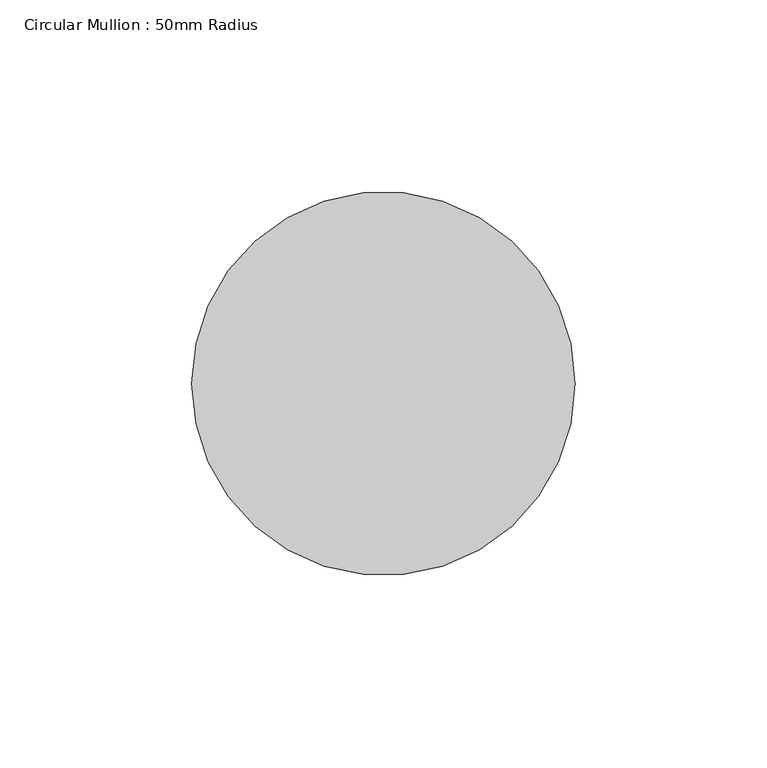
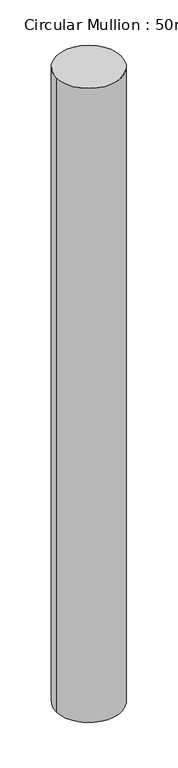
"""IFC4 building model written with IfcOpenShell, lengths in millimetres: member geometry, Circular Mullion : 50mm Radius."""

import ifcopenshell
import ifcopenshell.guid

model = None  # the IFC model being written
_history = None  # IfcOwnerHistory: only IFC2X3 demands one
_inside = {}  # id of a spatial element -> (the spatial element, [elements in it])
_under = {}  # id of a project, library or spatial element -> (it, [spatial elements below it])
_declared = {}  # id of a project -> (the project, [libraries it declares])
_typed = {}  # id of a type object -> (the type object, [elements of that type])
_made_of = {}  # id of a material, layer set ... -> (it, [elements and type objects made of it])


def new_model(schema):
    """Start an empty IFC model of exactly this schema.

    Asked for "IFC4X3", IfcOpenShell would pick the latest addendum, in which some entities
    have other attributes; the version numbers below select the first issue.
    IFC2X3 requires an IfcOwnerHistory on every rooted entity: one is made here for all.
    """
    global model, _history
    if schema == "IFC4X3":
        model = ifcopenshell.file(schema_version=(4, 3, 0, 0))
    else:
        model = ifcopenshell.file(schema=schema)
    _inside.clear()
    _under.clear()
    _declared.clear()
    _typed.clear()
    _made_of.clear()
    _history = None
    if model.schema == "IFC2X3":
        org = make("IfcOrganization", Name="unknown")
        user = make(
            "IfcPersonAndOrganization",
            ThePerson=make("IfcPerson", FamilyName="unknown"),
            TheOrganization=org,
        )
        app = make(
            "IfcApplication",
            ApplicationDeveloper=org,
            Version="unknown",
            ApplicationFullName="unknown",
            ApplicationIdentifier="unknown",
        )
        _history = make(
            "IfcOwnerHistory",
            OwningUser=user,
            OwningApplication=app,
            ChangeAction="ADDED",
            CreationDate=0,
        )
    return model


def make(cls, **values):
    """One entity of the class cls with the attributes given. An attribute that is None is left unset."""
    return model.create_entity(
        cls, **{name: value for name, value in values.items() if value is not None}
    )


def rooted(cls, **values):
    """An entity with a GlobalId (a new one), such as an element, a storey or a relation."""
    return make(cls, GlobalId=ifcopenshell.guid.new(), OwnerHistory=_history, **values)


def si_unit(unit_type, name, prefix=None):
    """IfcSIUnit, for example si_unit("LENGTHUNIT", "METRE", prefix="MILLI")."""
    return make("IfcSIUnit", UnitType=unit_type, Prefix=prefix, Name=name)


def assignment(units):
    """IfcUnitAssignment: the units of a project."""
    return None if units is None else make("IfcUnitAssignment", Units=units)


def point(xyz):
    """IfcCartesianPoint."""
    return None if xyz is None else make("IfcCartesianPoint", Coordinates=xyz)


def direction(xyz):
    """IfcDirection."""
    return None if xyz is None else make("IfcDirection", DirectionRatios=xyz)


def frame(location, z_axis=None, x_axis=None):
    """IfcAxis2Placement3D, a coordinate frame: its origin and axes. An axis left out is left unset."""
    return make(
        "IfcAxis2Placement3D",
        Location=point(location),
        Axis=direction(z_axis),
        RefDirection=direction(x_axis),
    )


def frame_2d(location, x_axis=None):
    """IfcAxis2Placement2D, a coordinate frame in the plane: its origin and x axis."""
    return make(
        "IfcAxis2Placement2D", Location=point(location), RefDirection=direction(x_axis)
    )


def origin():
    """The frame at (0, 0, 0) with its axes left unset."""
    return frame((0.0, 0.0, 0.0))


def origin_2d():
    """The frame at (0, 0) in the plane with its x axis left unset."""
    return frame_2d((0.0, 0.0))


def place(relative_to, where):
    """IfcLocalPlacement: puts the frame where relative to a parent placement (None: the world)."""
    return make(
        "IfcLocalPlacement", PlacementRelTo=relative_to, RelativePlacement=where
    )


def context(
    kind, dimensions, precision=None, world=None, true_north=None, identifier=None
):
    """IfcGeometricRepresentationContext, for example the 3D "Model" context."""
    return make(
        "IfcGeometricRepresentationContext",
        ContextIdentifier=identifier,
        ContextType=kind,
        CoordinateSpaceDimension=dimensions,
        Precision=precision,
        WorldCoordinateSystem=world,
        TrueNorth=true_north,
    )


def project(units=None, contexts=None):
    """IfcProject with its units and contexts."""
    return rooted(
        "IfcProject",
        Name="project",
        RepresentationContexts=contexts,
        UnitsInContext=assignment(units),
    )


def spatial(cls, under=None, at=None, **own):
    """A site, building, storey or space (cls), placed at a placement, below another one or the project."""
    s = rooted(cls, ObjectPlacement=at, **own)
    if under is not None:
        _under.setdefault(under.id(), (under, []))[1].append(s)
    return s


def circle_curve(where, radius):
    """IfcCircle in the frame where."""
    return make("IfcCircle", Position=where, Radius=radius)


def trimmed(basis, trim1, trim2, sense, master):
    """IfcTrimmedCurve: the piece of a basis curve between two trims."""
    return make(
        "IfcTrimmedCurve",
        BasisCurve=basis,
        Trim1=trim1,
        Trim2=trim2,
        SenseAgreement=sense,
        MasterRepresentation=master,
    )


def segment(curve, same_sense, transition):
    """IfcCompositeCurveSegment."""
    return make(
        "IfcCompositeCurveSegment",
        Transition=transition,
        SameSense=same_sense,
        ParentCurve=curve,
    )


def composite_curve(segments, self_intersect=None):
    """IfcCompositeCurve: segments joined end to end."""
    return make("IfcCompositeCurve", Segments=segments, SelfIntersect=self_intersect)


def outline(outer, holes=None, kind="AREA"):
    """IfcArbitraryClosedProfileDef: a profile drawn as a closed curve; with holes, ...WithVoids."""
    if holes is None:
        return make("IfcArbitraryClosedProfileDef", ProfileType=kind, OuterCurve=outer)
    return make(
        "IfcArbitraryProfileDefWithVoids",
        ProfileType=kind,
        OuterCurve=outer,
        InnerCurves=holes,
    )


def extrude(swept, where, along, depth):
    """IfcExtrudedAreaSolid: the profile swept, set in the frame where, extruded along a direction by depth."""
    return make(
        "IfcExtrudedAreaSolid",
        SweptArea=swept,
        Position=where,
        ExtrudedDirection=direction(along),
        Depth=depth,
    )


def shape(context_of_items, identifier, shape_type, items):
    """IfcShapeRepresentation: the items that make up one representation, for example the "Body"."""
    return make(
        "IfcShapeRepresentation",
        ContextOfItems=context_of_items,
        RepresentationIdentifier=identifier,
        RepresentationType=shape_type,
        Items=items,
    )


def source(mapping_origin, context_of_items, identifier, shape_type, items):
    """IfcRepresentationMap: a shape defined once, which mapped items show again and again."""
    return make(
        "IfcRepresentationMap",
        MappingOrigin=mapping_origin,
        MappedRepresentation=shape(context_of_items, identifier, shape_type, items),
    )


def transform(
    local_origin,
    x_axis=None,
    y_axis=None,
    z_axis=None,
    scale=None,
    scale2=None,
    scale3=None,
    uniform=True,
):
    """IfcCartesianTransformationOperator3D, or its non-uniform kind. x_axis, y_axis, z_axis: its Axis1, 2, 3."""
    if uniform:
        return make(
            "IfcCartesianTransformationOperator3D",
            Axis1=direction(x_axis),
            Axis2=direction(y_axis),
            LocalOrigin=point(local_origin),
            Scale=scale,
            Axis3=direction(z_axis),
        )
    return make(
        "IfcCartesianTransformationOperator3DnonUniform",
        Axis1=direction(x_axis),
        Axis2=direction(y_axis),
        LocalOrigin=point(local_origin),
        Scale=scale,
        Axis3=direction(z_axis),
        Scale2=scale2,
        Scale3=scale3,
    )


def mapped(mapping_source, mapping_target):
    """IfcMappedItem: shows the shape of a source again, moved by a transform."""
    return make(
        "IfcMappedItem", MappingSource=mapping_source, MappingTarget=mapping_target
    )


def made_of(thing, what):
    """Note that an element or type object is made of a material, layer set ...; save() writes the relation."""
    if what is not None:
        _made_of.setdefault(what.id(), (what, []))[1].append(thing)
    return thing


def element(
    cls,
    number,
    at=None,
    inside=None,
    cuts=None,
    type_object=None,
    material=None,
    context=None,
    identifier="Body",
    shape_type=None,
    held_by="IfcProductDefinitionShape",
    body=None,
    shapes=None,
    **own,
):
    """One element of the class cls, such as IfcWall. Its Tag is "e" and its number.

    at: its placement. inside: the storey or other place that contains it. cuts: it is an
    opening in that element (IfcRelVoidsElement). A single representation is given by context,
    identifier, shape_type and body (its items); several are given by shapes. held_by: the class
    of the entity that holds the representations. save() writes the other relations.
    """
    e = rooted(cls, Tag="e%d" % number, ObjectPlacement=at, **own)
    if body is not None:
        shapes = [shape(context, identifier, shape_type, body)]
    if shapes is not None:
        e.Representation = make(held_by, Representations=shapes)
    if inside is not None:
        _inside.setdefault(inside.id(), (inside, []))[1].append(e)
    if cuts is not None:
        rooted(
            "IfcRelVoidsElement", RelatingBuildingElement=cuts, RelatedOpeningElement=e
        )
    if type_object is not None:
        _typed.setdefault(type_object.id(), (type_object, []))[1].append(e)
    return made_of(e, material)


def aggregate(whole, parts):
    """IfcRelAggregates: a whole, such as a stair, and the parts it consists of."""
    return rooted("IfcRelAggregates", RelatingObject=whole, RelatedObjects=parts)


def save(model, path):
    """Write the relations noted so far, then the file.

    IfcRelAggregates (storeys below a building ...), IfcRelContainedInSpatialStructure (elements
    in a storey), IfcRelDefinesByType, IfcRelAssociatesMaterial and IfcRelDeclares: one each for
    every whole, place, type object, material and project.
    """
    for whole, parts in _under.values():
        aggregate(whole, parts)
    for where, things in _inside.values():
        rooted(
            "IfcRelContainedInSpatialStructure",
            RelatedElements=things,
            RelatingStructure=where,
        )
    for kind, things in _typed.values():
        rooted("IfcRelDefinesByType", RelatedObjects=things, RelatingType=kind)
    for what, things in _made_of.values():
        rooted("IfcRelAssociatesMaterial", RelatedObjects=things, RelatingMaterial=what)
    for by, libraries in _declared.values():
        rooted("IfcRelDeclares", RelatingContext=by, RelatedDefinitions=libraries)
    model.write(path)


def circular_mullion_50mm_radius_73201df1(model_context):
    return source(origin(), model_context, "Body", "SweptSolid", [
        extrude(outline(composite_curve([segment(trimmed(circle_curve(origin_2d(), 50.0), [point((50.0, 0.0))], [point((-50.0, 0.0))], False, "CARTESIAN"), True, "CONTINUOUS"), segment(trimmed(circle_curve(origin_2d(), 50.0), [point((-50.0, 0.0))], [point((50.0, 0.0))], False, "CARTESIAN"), True, "CONTINUOUS")], self_intersect=False)), frame((0.0, 0.0, -1031.9932512), z_axis=(0.0, 0.0, 1.0), x_axis=(1.0, 0.0, 0.0)), (0.0, 0.0, 1.0), 1031.9932512),
    ])


if __name__ == "__main__":
    model = new_model("IFC4")
    model_context = context("Model", 3, world=origin())
    ifc_project = project(units=[si_unit("LENGTHUNIT", "METRE", prefix="MILLI")], contexts=[model_context])
    site = spatial("IfcSite", under=ifc_project)
    building = spatial("IfcBuilding", under=site)
    placement = place(None, origin())
    circular_mullion_50mm_radius_shape = circular_mullion_50mm_radius_73201df1(model_context)
    element("IfcMember", 1, ObjectType="Circular Mullion : 50mm Radius", at=placement, inside=building, context=model_context, shape_type="MappedRepresentation", body=[
        mapped(circular_mullion_50mm_radius_shape, transform((0.0, 0.0, 0.0), x_axis=(1.0, 0.0, 0.0), y_axis=(0.0, 1.0, 0.0), z_axis=(0.0, 0.0, 1.0))),
    ])
    save(model, "model.ifc")

# Revit data of these elements
# Type "Circular Mullion : 50mm Radius"
#   built-in parameter 1007350 = 0.164042 (stored number, unit not read)
# Element 1 (IfcMember, "Circular Mullion : 50mm Radius")
#   Materials on its faces: "Aluminium"
# Materials
#   "Aluminium": class "Metal", colour RGB 247 247 247, transparency 0, Description = "Aluminium 6061", Cost = 0
